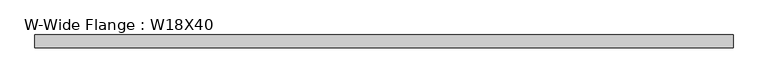
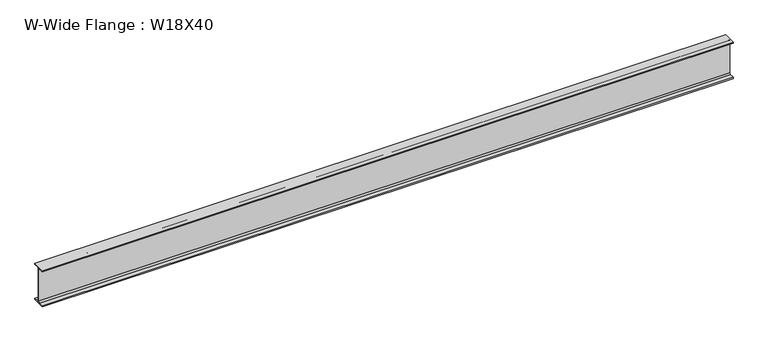
"""IFC4 building model written with IfcOpenShell, lengths in millimetres: beam geometry, W-Wide Flange : W18X40."""

from ifc_helpers import new_model, si_unit, point, frame, frame_2d, origin, place, context, project, spatial, polyline, circle_curve, trimmed, segment, composite_curve, outline, extrude, source, transform, mapped, element, save


def w_wide_flange_w18x40_897d76ae(model_context):
    return source(origin(), model_context, "Body", "SweptSolid", [
        extrude(outline(composite_curve([segment(polyline([(76.454, -213.995), (76.454, -227.33), (-76.454, -227.33), (-76.454, -213.995), (-20.828, -213.995)]), True, "CONTINUOUS"), segment(trimmed(circle_curve(frame_2d((-20.828, -197.1675)), 16.8275), [point((-20.828, -213.995))], [point((-4.0005, -197.1675))], True, "CARTESIAN"), True, "CONTINUOUS"), segment(polyline([(-4.0005, -197.1675), (-4.0005, 197.1675)]), True, "CONTINUOUS"), segment(trimmed(circle_curve(frame_2d((-20.828, 197.1675)), 16.8275), [point((-4.0005, 197.1675))], [point((-20.828, 213.995))], True, "CARTESIAN"), True, "CONTINUOUS"), segment(polyline([(-20.828, 213.995), (-76.454, 213.995), (-76.454, 227.33), (76.454, 227.33), (76.454, 213.995), (20.828, 213.995)]), True, "CONTINUOUS"), segment(trimmed(circle_curve(frame_2d((20.828, 197.1675)), 16.8275), [point((20.828, 213.995))], [point((4.0005, 197.1675))], True, "CARTESIAN"), True, "CONTINUOUS"), segment(polyline([(4.0005, 197.1675), (4.0005, -197.1675)]), True, "CONTINUOUS"), segment(trimmed(circle_curve(frame_2d((20.828, -197.1675)), 16.8275), [point((4.0005, -197.1675))], [point((20.828, -213.995))], True, "CARTESIAN"), True, "CONTINUOUS"), segment(polyline([(20.828, -213.995), (76.454, -213.995)]), True, "CONTINUOUS")], self_intersect=False)), frame((-4100.83, 0.0, 0.0), z_axis=(1.0, 0.0, 0.0), x_axis=(0.0, 1.0, 0.0)), (0.0, 0.0, 1.0), 8201.66),
    ])


if __name__ == "__main__":
    model = new_model("IFC4")
    model_context = context("Model", 3, world=origin())
    ifc_project = project(units=[si_unit("LENGTHUNIT", "METRE", prefix="MILLI")], contexts=[model_context])
    site = spatial("IfcSite", under=ifc_project)
    building = spatial("IfcBuilding", under=site)
    placement = place(None, origin())
    w_wide_flange_w18x40_shape = w_wide_flange_w18x40_897d76ae(model_context)
    element("IfcBeam", 1, ObjectType="W-Wide Flange : W18X40", at=placement, inside=building, context=model_context, shape_type="MappedRepresentation", body=[
        mapped(w_wide_flange_w18x40_shape, transform((0.0, 0.0, 0.0), x_axis=(1.0, 0.0, 0.0), y_axis=(0.0, 1.0, 0.0), z_axis=(0.0, 0.0, 1.0))),
    ])
    save(model, "model.ifc")

# Revit data of these elements
# Type "W-Wide Flange : W18X40"
#   Assembly Code = "B10"
#   W = 40
#   Length [instance default] = 5' - 0"
#   bf = 0' - 6.02"
#   d = 1' - 5.9"
#   k = 0' - 1 3/16"
#   k2 = 0' - 0.6625"
#   tf = 0' - 0.525"
#   tw = 0' - 0.315"
#   A = 0.0819444 SF
#   Structural Material [instance default] = Steel ASTM A992
# Element 1 (IfcBeam, "W-Wide Flange : W18X40")
#   Materials on its faces: "Steel ASTM A992"
# Materials
#   "Steel ASTM A992": class "Metal", colour RGB 199 199 199, transparency 0, Description = "Structural steel 50ksi", Cost = 0
